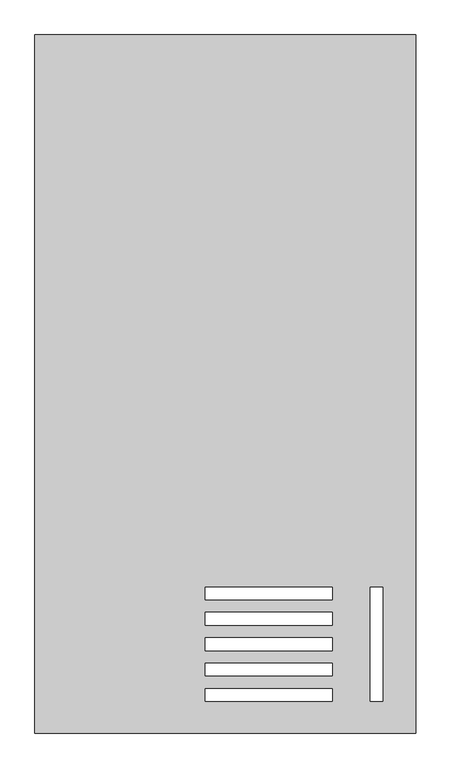
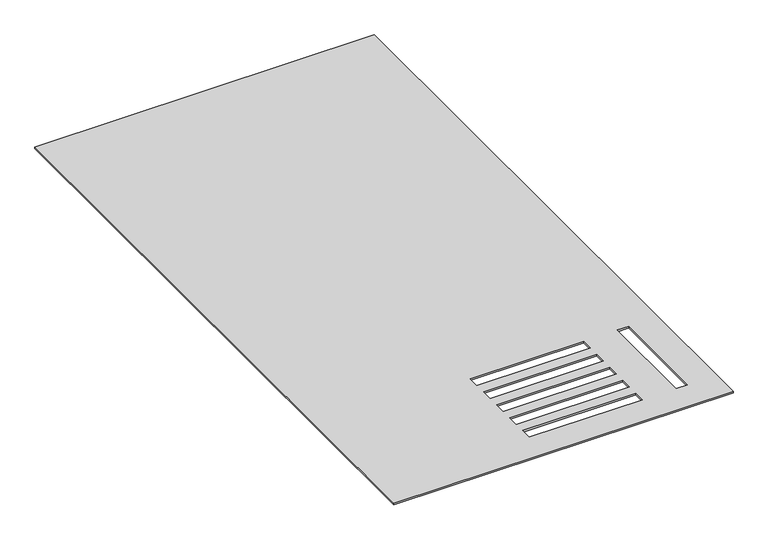
"""IFC4 building model written with IfcOpenShell, lengths in millimetres: proxy geometry, TSP Geyser Solar 150L : TSP Geyser Solar 150L."""

from ifc_helpers import new_model, si_unit, origin, origin_with_axes, place, context, project, spatial, polyline, outline, extrude, source, transform, mapped, element, save


def electrical_fixtures_8066117e(model_context):
    return source(origin(), model_context, "Body", "SweptSolid", [
        extrude(outline(polyline([(-600.0, 600.0), (0.0, 600.0), (0.0, -500.0), (-600.0, -500.0), (-600.0, 600.0)]), holes=[polyline([(-71.8082825, -450.0), (-51.8082825, -450.0), (-51.8082825, -270.0), (-71.8082825, -270.0), (-71.8082825, -450.0)]), polyline([(-131.8082825, -270.0), (-331.8082825, -270.0), (-331.8082825, -290.0), (-131.8082825, -290.0), (-131.8082825, -270.0)]), polyline([(-131.8082825, -310.0), (-331.8082825, -310.0), (-331.8082825, -330.0), (-131.8082825, -330.0), (-131.8082825, -310.0)]), polyline([(-131.8082825, -350.0), (-331.8082825, -350.0), (-331.8082825, -370.0), (-131.8082825, -370.0), (-131.8082825, -350.0)]), polyline([(-131.8082825, -390.0), (-331.8082825, -390.0), (-331.8082825, -410.0), (-131.8082825, -410.0), (-131.8082825, -390.0)]), polyline([(-131.8082825, -430.0), (-331.8082825, -430.0), (-331.8082825, -450.0), (-131.8082825, -450.0), (-131.8082825, -430.0)])]), origin_with_axes(), (0.0, 0.0, 1.0), 3.0),
    ])


if __name__ == "__main__":
    model = new_model("IFC4")
    model_context = context("Model", 3, world=origin())
    ifc_project = project(units=[si_unit("LENGTHUNIT", "METRE", prefix="MILLI")], contexts=[model_context])
    site = spatial("IfcSite", under=ifc_project)
    building = spatial("IfcBuilding", under=site)
    placement = place(None, origin())
    electrical_fixtures_shape = electrical_fixtures_8066117e(model_context)
    element("IfcBuildingElementProxy", 1, Name="TSP Geyser Solar 150L : TSP Geyser Solar 150L", ObjectType="TSP Geyser Solar 150L : TSP Geyser Solar 150L", at=placement, inside=building, context=model_context, shape_type="MappedRepresentation", body=[
        mapped(electrical_fixtures_shape, transform((0.0, 0.0, 0.0), x_axis=(1.0, 0.0, 0.0), y_axis=(0.0, 1.0, 0.0), z_axis=(0.0, 0.0, 1.0))),
    ])
    save(model, "model.ifc")

# Revit data of these elements
# Type "TSP Geyser Solar 150L : TSP Geyser Solar 150L"
#   Model = "TSP_SGEY150"
#   Default Elevation = 0
# Element 1 (IfcBuildingElementProxy, "TSP Geyser Solar 150L : TSP Geyser Solar 150L")
#   Materials on its faces: "Aluminum, Anodized Red"
# Materials
#   "Aluminum, Anodized Red": class "Metal", colour RGB 120 120 120, transparency 0, Description = "Anodized aluminum, red", Cost = 0
